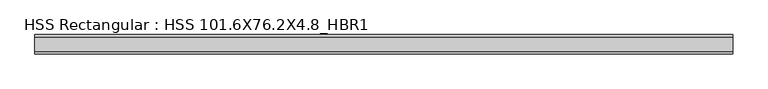
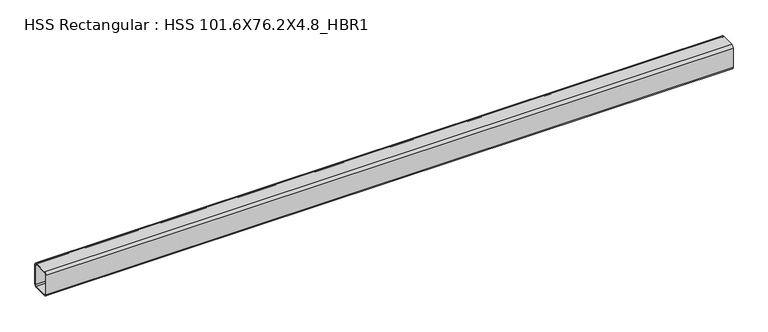
"""IFC4 building model written with IfcOpenShell, lengths in millimetres: beam geometry, HSS Rectangular : HSS 101.6X76.2X4.8_HBR1."""

from ifc_helpers import new_model, si_unit, point, frame, frame_2d, origin, place, context, project, spatial, polyline, circle_curve, trimmed, segment, composite_curve, outline, extrude, source, transform, mapped, element, save


def hss_rectangular_hss_101_6x76_2x4_8_hbr1_73f01b4a(model_context):
    return source(origin(), model_context, "Body", "SweptSolid", [
        extrude(outline(composite_curve([segment(polyline([(38.1, 41.275), (38.1, -41.275)]), True, "CONTINUOUS"), segment(trimmed(circle_curve(frame_2d((28.575, -41.275)), 9.525), [point((38.1, -41.275))], [point((28.575, -50.8))], False, "CARTESIAN"), True, "CONTINUOUS"), segment(polyline([(28.575, -50.8), (-28.575, -50.8)]), True, "CONTINUOUS"), segment(trimmed(circle_curve(frame_2d((-28.575, -41.275)), 9.525), [point((-28.575, -50.8))], [point((-38.1, -41.275))], False, "CARTESIAN"), True, "CONTINUOUS"), segment(polyline([(-38.1, -41.275), (-38.1, 41.275)]), True, "CONTINUOUS"), segment(trimmed(circle_curve(frame_2d((-28.575, 41.275)), 9.525), [point((-38.1, 41.275))], [point((-28.575, 50.8))], False, "CARTESIAN"), True, "CONTINUOUS"), segment(polyline([(-28.575, 50.8), (28.575, 50.8)]), True, "CONTINUOUS"), segment(trimmed(circle_curve(frame_2d((28.575, 41.275)), 9.525), [point((28.575, 50.8))], [point((38.1, 41.275))], False, "CARTESIAN"), True, "CONTINUOUS")], self_intersect=False), holes=[composite_curve([segment(trimmed(circle_curve(frame_2d((-28.575, 41.275)), 4.7625), [point((-28.575, 46.0375))], [point((-33.3375, 41.275))], True, "CARTESIAN"), True, "CONTINUOUS"), segment(polyline([(-33.3375, 41.275), (-33.3375, -41.275)]), True, "CONTINUOUS"), segment(trimmed(circle_curve(frame_2d((-28.575, -41.275)), 4.7625), [point((-33.3375, -41.275))], [point((-28.575, -46.0375))], True, "CARTESIAN"), True, "CONTINUOUS"), segment(polyline([(-28.575, -46.0375), (28.575, -46.0375)]), True, "CONTINUOUS"), segment(trimmed(circle_curve(frame_2d((28.575, -41.275)), 4.7625), [point((28.575, -46.0375))], [point((33.3375, -41.275))], True, "CARTESIAN"), True, "CONTINUOUS"), segment(polyline([(33.3375, -41.275), (33.3375, 41.275)]), True, "CONTINUOUS"), segment(trimmed(circle_curve(frame_2d((28.575, 41.275)), 4.7625), [point((33.3375, 41.275))], [point((28.575, 46.0375))], True, "CARTESIAN"), True, "CONTINUOUS"), segment(polyline([(28.575, 46.0375), (-28.575, 46.0375)]), True, "CONTINUOUS")], self_intersect=False)]), frame((-1390.6637409, 0.0, 0.0), z_axis=(1.0, 0.0, 0.0), x_axis=(0.0, 1.0, 0.0)), (0.0, 0.0, 1.0), 2762.2264788),
    ])


if __name__ == "__main__":
    model = new_model("IFC4")
    model_context = context("Model", 3, world=origin())
    ifc_project = project(units=[si_unit("LENGTHUNIT", "METRE", prefix="MILLI")], contexts=[model_context])
    site = spatial("IfcSite", under=ifc_project)
    building = spatial("IfcBuilding", under=site)
    placement = place(None, origin())
    hss_rectangular_hss_101_6x76_2x4_8_hbr1_shape = hss_rectangular_hss_101_6x76_2x4_8_hbr1_73f01b4a(model_context)
    element("IfcBeam", 1, ObjectType="HSS Rectangular : HSS 101.6X76.2X4.8_HBR1", at=placement, inside=building, context=model_context, shape_type="MappedRepresentation", body=[
        mapped(hss_rectangular_hss_101_6x76_2x4_8_hbr1_shape, transform((0.0, 0.0, 0.0), x_axis=(1.0, 0.0, 0.0), y_axis=(0.0, 1.0, 0.0), z_axis=(0.0, 0.0, 1.0))),
    ])
    save(model, "model.ifc")

# Revit data of these elements
# Type "HSS Rectangular : HSS 101.6X76.2X4.8_HBR1"
#   Section Name Key = "HSS 4X3X3/16"
#   Assembly Code = "B10"
#   Width = 7.62 cm
#   Wall Nominal Thickness = 0.4763 cm
#   Wall Design Thickness = 0.442 cm
#   Torsional Moment of Inertia = 260.561 cm⁴
#   Torsional Modulus = 61.2876 cm³
#   Section Area = 14.4516 cm²
#   Plastic Modulus weak axis = 40.3122 cm³
#   Plastic Modulus strong axis = 49.1612 cm³
#   Perimeter = 0.881482 m²/m
#   Outer Fillet = 0.9525 cm
#   Nominal Weight = 12.1285 kgf/m
#   Moment of Inertia weak axis = 131.529 cm⁴
#   Moment of Inertia strong axis = 205.202 cm⁴
#   Inner Fillet = 0.4763 cm
#   Height = 10.16 cm
#   Elastic Modulus weak axis = 34.4128 cm³
#   Elastic Modulus strong axis = 40.476 cm³
#   Centroid Vertical = 5.08 cm
#   Centroid Horizontal = 3.81 cm
#   Length [instance default] = 1524 mm
#   Structural Material [instance default] = Steel ASTM A500, Grade B, Rectangular and Square
#   Principal Axes Angle = 0
# Element 1 (IfcBeam, "HSS Rectangular : HSS 101.6X76.2X4.8_HBR1")
#   Structural Material = Steel ASTM A992
#   Materials on its faces: "Steel ASTM A992"
# Materials
#   "Steel ASTM A500, Grade B, Rectangular and Square": class "Metal", colour RGB 199 199 199, transparency 0, Description = "Carbon steel", Cost = 0
#   "Steel ASTM A992": class "Metal", colour RGB 199 199 199, transparency 0, Description = "Structural steel 50ksi", Cost = 0
